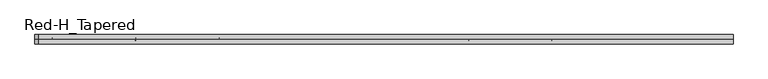
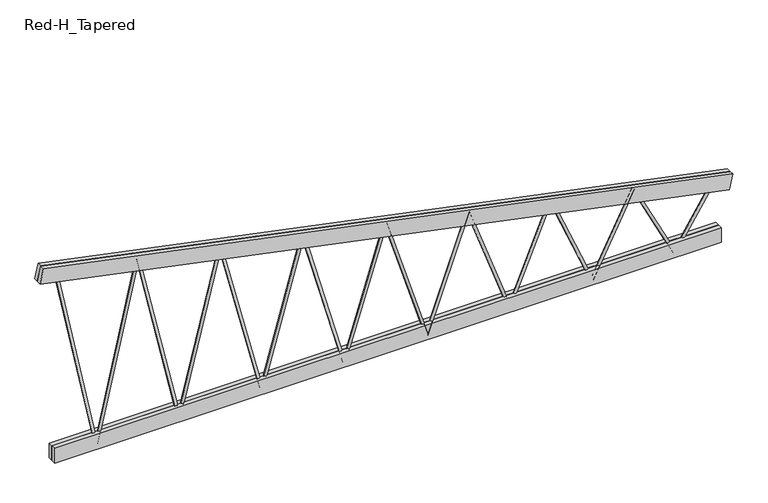
"""IFC4 building model written with IfcOpenShell, lengths in millimetres: beam geometry, Construction_Frames_RedBuilt_Openweb_Red-H_Tapered : Red-H_Tapered."""

from ifc_helpers import new_model, si_unit, point, frame, origin, origin_2d, place, context, project, spatial, polyline, circle_curve, trimmed, segment, composite_curve, outline, extrude, source, transform, mapped, element, save


def red_h_tapered_cb119500(model_context):
    return source(origin(), model_context, "Body", "SweptSolid", [
        extrude(outline(composite_curve([segment(trimmed(circle_curve(origin_2d(), 12.7), [point((0.0, 12.7))], [point((0.0, -12.7))], False, "CARTESIAN"), True, "CONTINUOUS"), segment(trimmed(circle_curve(origin_2d(), 12.7), [point((0.0, -12.7))], [point((0.0, 12.7))], False, "CARTESIAN"), True, "CONTINUOUS")], self_intersect=False)), frame((-368.7971472, 0.0, -367.0101562), z_axis=(-0.26750269153884754, 0.0, 0.9635571130034131), x_axis=(0.0, -1.0, 0.0)), (0.0, 0.0, 1.0), 1378.6670521),
        extrude(outline(composite_curve([segment(trimmed(circle_curve(origin_2d(), 12.7), [point((0.0, -12.7))], [point((0.0, 12.7))], False, "CARTESIAN"), True, "CONTINUOUS"), segment(trimmed(circle_curve(origin_2d(), 12.7), [point((0.0, 12.7))], [point((0.0, -12.7))], False, "CARTESIAN"), True, "CONTINUOUS")], self_intersect=False)), frame((-1106.3914415, 0.0, -367.0101562), z_axis=(0.2675026915388467, 0.0, 0.9635571130034134), x_axis=(0.0, -1.0, 0.0)), (0.0, 0.0, 1.0), 1378.6670521),
        extrude(outline(composite_curve([segment(trimmed(circle_curve(origin_2d(), 12.7), [point((0.0, 12.6999999))], [point((0.0, -12.7))], False, "CARTESIAN"), True, "CONTINUOUS"), segment(trimmed(circle_curve(origin_2d(), 12.7), [point((0.0, -12.7))], [point((0.0, 12.6999999))], False, "CARTESIAN"), True, "CONTINUOUS")], self_intersect=False)), frame((-1106.3914415, 0.0, -367.0101562), z_axis=(-0.2422140667731756, 0.0, 0.9702228330941298), x_axis=(0.0, -1.0, 0.0)), (0.0, 0.0, 1.0), 1522.6082948),
        extrude(outline(composite_curve([segment(trimmed(circle_curve(origin_2d(), 12.7), [point((0.0, -12.7))], [point((0.0, 12.7))], False, "CARTESIAN"), True, "CONTINUOUS"), segment(trimmed(circle_curve(origin_2d(), 12.7), [point((0.0, 12.7))], [point((0.0, -12.7))], False, "CARTESIAN"), True, "CONTINUOUS")], self_intersect=False)), frame((-1843.9857359, 0.0, -367.0101562), z_axis=(0.2422140667731837, 0.0, 0.9702228330941278), x_axis=(0.0, -1.0, 0.0)), (0.0, 0.0, 1.0), 1522.6082948),
        extrude(outline(composite_curve([segment(trimmed(circle_curve(origin_2d(), 12.7), [point((0.0, 12.7))], [point((0.0, -12.7))], False, "CARTESIAN"), True, "CONTINUOUS"), segment(trimmed(circle_curve(origin_2d(), 12.7), [point((0.0, -12.7))], [point((0.0, 12.7))], False, "CARTESIAN"), True, "CONTINUOUS")], self_intersect=False)), frame((-1843.9857359, 0.0, -367.0101562), z_axis=(-0.22117953511549954, 0.0, 0.9752331071318752), x_axis=(0.0, -1.0, 0.0)), (0.0, 0.0, 1.0), 1667.4108072),
        extrude(outline(composite_curve([segment(trimmed(circle_curve(origin_2d(), 12.7), [point((0.0, -12.6999999))], [point((0.0, 12.7))], False, "CARTESIAN"), True, "CONTINUOUS"), segment(trimmed(circle_curve(origin_2d(), 12.7), [point((0.0, 12.7))], [point((0.0, -12.6999999))], False, "CARTESIAN"), True, "CONTINUOUS")], self_intersect=False)), frame((-2581.5800303, 0.0, -367.0101562), z_axis=(0.22117953511549293, 0.0, 0.9752331071318767), x_axis=(0.0, -1.0, 0.0)), (0.0, 0.0, 1.0), 1667.4108072),
        extrude(outline(composite_curve([segment(trimmed(circle_curve(origin_2d(), 12.7), [point((0.0, 12.7))], [point((0.0, -12.7))], False, "CARTESIAN"), True, "CONTINUOUS"), segment(trimmed(circle_curve(origin_2d(), 12.7), [point((0.0, -12.7))], [point((0.0, 12.7))], False, "CARTESIAN"), True, "CONTINUOUS")], self_intersect=False)), frame((-2581.5800303, 0.0, -367.0101562), z_axis=(-0.2034329595212491, 0.0, 0.9790888779781056), x_axis=(0.0, -1.0, 0.0)), (0.0, 0.0, 1.0), 1812.8682198),
        extrude(outline(composite_curve([segment(trimmed(circle_curve(origin_2d(), 12.7), [point((0.0, 12.7))], [point((0.0, -12.7))], False, "CARTESIAN"), True, "CONTINUOUS"), segment(trimmed(circle_curve(origin_2d(), 12.7), [point((0.0, -12.7))], [point((0.0, 12.7))], False, "CARTESIAN"), True, "CONTINUOUS")], self_intersect=False)), frame((2581.5800303, 0.0, -367.0101562), z_axis=(0.5338157604547286, 0.0, 0.8456008123755203), x_axis=(0.0, -1.0, 0.0)), (0.0, 0.0, 1.0), 690.8697242),
        extrude(outline(composite_curve([segment(trimmed(circle_curve(origin_2d(), 12.7), [point((0.0, -12.7000001))], [point((0.0, 12.6999999))], False, "CARTESIAN"), True, "CONTINUOUS"), segment(trimmed(circle_curve(origin_2d(), 12.7), [point((0.0, 12.6999999))], [point((0.0, -12.7000001))], False, "CARTESIAN"), True, "CONTINUOUS")], self_intersect=False)), frame((2581.5800303, 0.0, -367.0101562), z_axis=(-0.4494298504402509, 0.0, 0.8933156270508502), x_axis=(0.0, -1.0, 0.0)), (0.0, 0.0, 1.0), 820.5889013),
        extrude(outline(composite_curve([segment(trimmed(circle_curve(origin_2d(), 12.7), [point((0.0, 12.7000001))], [point((0.0, -12.7))], False, "CARTESIAN"), True, "CONTINUOUS"), segment(trimmed(circle_curve(origin_2d(), 12.7), [point((0.0, -12.7))], [point((0.0, 12.7000001))], False, "CARTESIAN"), True, "CONTINUOUS")], self_intersect=False)), frame((1843.9857359, 0.0, -367.0101562), z_axis=(0.44942985044025024, 0.0, 0.8933156270508507), x_axis=(0.0, -1.0, 0.0)), (0.0, 0.0, 1.0), 820.5889013),
        extrude(outline(composite_curve([segment(trimmed(circle_curve(origin_2d(), 12.7), [point((0.0, -12.7))], [point((0.0, 12.7))], False, "CARTESIAN"), True, "CONTINUOUS"), segment(trimmed(circle_curve(origin_2d(), 12.7), [point((0.0, 12.7))], [point((0.0, -12.7))], False, "CARTESIAN"), True, "CONTINUOUS")], self_intersect=False)), frame((1843.9857359, 0.0, -367.0101562), z_axis=(-0.38581225339019065, 0.0, 0.9225773166157856), x_axis=(0.0, -1.0, 0.0)), (0.0, 0.0, 1.0), 955.8979632),
        extrude(outline(composite_curve([segment(trimmed(circle_curve(origin_2d(), 12.7), [point((0.0, 12.7000001))], [point((0.0, -12.7))], False, "CARTESIAN"), True, "CONTINUOUS"), segment(trimmed(circle_curve(origin_2d(), 12.7), [point((0.0, -12.7))], [point((0.0, 12.7000001))], False, "CARTESIAN"), True, "CONTINUOUS")], self_intersect=False)), frame((1106.3914415, 0.0, -367.0101562), z_axis=(0.38581225339018976, 0.0, 0.9225773166157859), x_axis=(0.0, -1.0, 0.0)), (0.0, 0.0, 1.0), 955.8979632),
        extrude(outline(composite_curve([segment(trimmed(circle_curve(origin_2d(), 12.7), [point((0.0, -12.7))], [point((0.0, 12.7))], False, "CARTESIAN"), True, "CONTINUOUS"), segment(trimmed(circle_curve(origin_2d(), 12.7), [point((0.0, 12.7))], [point((0.0, -12.7))], False, "CARTESIAN"), True, "CONTINUOUS")], self_intersect=False)), frame((1106.3914415, 0.0, -367.0101562), z_axis=(-0.3368853074093003, 0.0, 0.9415456917493391), x_axis=(0.0, -1.0, 0.0)), (0.0, 0.0, 1.0), 1094.7261251),
        extrude(outline(composite_curve([segment(trimmed(circle_curve(origin_2d(), 12.7), [point((0.0, 12.7))], [point((0.0, -12.7))], False, "CARTESIAN"), True, "CONTINUOUS"), segment(trimmed(circle_curve(origin_2d(), 12.7), [point((0.0, -12.7))], [point((0.0, 12.7))], False, "CARTESIAN"), True, "CONTINUOUS")], self_intersect=False)), frame((368.7971472, 0.0, -367.0101562), z_axis=(0.33688530740930067, 0.0, 0.9415456917493389), x_axis=(0.0, -1.0, 0.0)), (0.0, 0.0, 1.0), 1094.7261251),
        extrude(outline(composite_curve([segment(trimmed(circle_curve(origin_2d(), 12.7), [point((0.0, -12.7))], [point((0.0, 12.7))], False, "CARTESIAN"), True, "CONTINUOUS"), segment(trimmed(circle_curve(origin_2d(), 12.7), [point((0.0, 12.7))], [point((0.0, -12.7))], False, "CARTESIAN"), True, "CONTINUOUS")], self_intersect=False)), frame((368.7971472, 0.0, -367.0101562), z_axis=(-0.29840659773502576, 0.0, 0.9544388416384816), x_axis=(0.0, -1.0, 0.0)), (0.0, 0.0, 1.0), 1235.8880466),
        extrude(outline(composite_curve([segment(trimmed(circle_curve(origin_2d(), 12.7), [point((0.0, -12.7))], [point((0.0, 12.7))], False, "CARTESIAN"), True, "CONTINUOUS"), segment(trimmed(circle_curve(origin_2d(), 12.7), [point((0.0, 12.7))], [point((0.0, -12.7))], False, "CARTESIAN"), True, "CONTINUOUS")], self_intersect=False)), frame((-368.7971472, 0.0, -367.0101562), z_axis=(0.29840659773500394, 0.0, 0.9544388416384885), x_axis=(0.0, -1.0, 0.0)), (0.0, 0.0, 1.0), 1235.8880466),
        extrude(outline(polyline([(-2975.7771774, -41.275), (-2975.7771774, -3.175), (2975.7771774, -3.175), (2975.7771774, -41.275), (-2975.7771774, -41.275)])), frame((0.0, 0.0, -386.0601562), z_axis=(0.0, 0.0, 1.0), x_axis=(1.0, 0.0, 0.0)), (0.0, 0.0, 1.0), 139.7),
        extrude(outline(polyline([(-2975.7771774, 3.175), (-2975.7771774, 41.275), (2975.7771774, 41.275), (2975.7771774, 3.175), (-2975.7771774, 3.175)])), frame((0.0, 0.0, -386.0601562), z_axis=(0.0, 0.0, 1.0), x_axis=(1.0, 0.0, 0.0)), (0.0, 0.0, 1.0), 139.7),
        extrude(outline(polyline([(0.0, -38.1), (0.0, 0.0), (6282.8180718, 0.0), (6282.8180718, -38.1), (0.0, -38.1)])), frame((-3105.4394465, -3.175, 1348.7498719), z_axis=(0.20087522598673502, 0.0, 0.9796168350864425), x_axis=(0.9796168350864425, 0.0, -0.20087522598673502)), (0.0, 0.0, 1.0), 139.7),
        extrude(outline(polyline([(0.0, -38.1), (0.0, 0.0), (6282.8180718, 0.0), (6282.8180718, -38.1), (0.0, -38.1)])), frame((-3105.4394465, 41.275, 1348.7498719), z_axis=(0.20087522598673502, 0.0, 0.9796168350864425), x_axis=(0.9796168350864425, 0.0, -0.20087522598673502)), (0.0, 0.0, 1.0), 139.7),
    ])


if __name__ == "__main__":
    model = new_model("IFC4")
    model_context = context("Model", 3, world=origin())
    ifc_project = project(units=[si_unit("LENGTHUNIT", "METRE", prefix="MILLI")], contexts=[model_context])
    site = spatial("IfcSite", under=ifc_project)
    building = spatial("IfcBuilding", under=site)
    placement = place(None, origin())
    red_h_tapered_shape = red_h_tapered_cb119500(model_context)
    element("IfcBeam", 1, ObjectType="Construction_Frames_RedBuilt_Openweb_Red-H_Tapered : Red-H_Tapered", at=placement, inside=building, context=model_context, shape_type="MappedRepresentation", body=[
        mapped(red_h_tapered_shape, transform((0.0, 0.0, 0.0), x_axis=(1.0, 0.0, 0.0), y_axis=(0.0, 1.0, 0.0), z_axis=(0.0, 0.0, 1.0))),
    ])
    save(model, "model.ifc")

# Revit data of these elements
# Type "Construction_Frames_RedBuilt_Openweb_Red-H_Tapered : Red-H_Tapered"
#   Youtube clip = ""
#   Weight Net (Kg) = "0"
#   Webs = "Up to 2\" diameter tubular steel"
#   Uniformat II Description = ""
#   Uniformat II Code = ""
#   Uniclass 2015 Name = "Softwood trusses"
#   Uniclass 2015 Code = "Pr_20_85_90_81"
#   Uniclass 2.0 Description = "Structural Framing Systems"
#   Uniclass 2.0 Code = "SS-15-10-75"
#   Uniclass 1.4 Description = "Trusses"
#   Uniclass 1.4 Code = "L3523"
#   UNSPSC Code = "30103606"
#   Technical description = "http://www.redbuilt.com/reference/literature-and-other-resources"
#   Region South America = "None"
#   Region Oceania = "None"
#   Region North America = "US"
#   Region Middle East = "None"
#   Region Europe = "None"
#   Region Asia = "None"
#   Region Antarctica = "None"
#   Region Africa = "None"
#   QR code = "http://bimobject.com/redbuilt/product/redbuilt-0003"
#   Product url = "http://www.redbuilt.com/products/default.aspx?id=2"
#   Product group = "Wood Trusses"
#   Product family = "Construction"
#   Product data url = "https://bimobject.com/redbuilt/product/redbuilt-0003"
#   Product certification = ""
#   Product SKU = "redbuilt-0003"
#   Product Page URL = "http://www.redbuilt.com/commercial-systems/red-m-red-h-open-web-trusses"
#   Product Guid = "2c5793f2-6ffb-4665-b825-cf90c048e711"
#   Product Documentation Link = "http://www.redbuilt.com/documents/OW_Guide_2017_07_LowRes_wLinks.pdf"
#   OmniClass Description = "Wood Trusses"
#   OmniClass Code = "23-13 35 19 13 17"
#   NBS Reference Description = ""
#   NBS Reference Code = ""
#   Material secondary = "Steel"
#   Material main = "Wood"
#   Masterformat 2014 Description = "Metal-Web Wood Joists"
#   Masterformat 2014 Code = "06 17 36"
#   Manufacturer name = "RedBuilt"
#   Manufacturer country = "United States"
#   Installation instructions = "http://www.redbuilt.com/documents/Installation_Sheets_Open-Web.pdf"
#   IFC Classification = ""
#   EAN code = ""
#   Design country = "United States"
#   Product Information = "http://redbuilt.com/products/default.aspx?id=2"
#   Model = "Red-H-Tapered"
#   Manufacturer URL = "http://redbuilt.com/"
#   Manufacturer = "RedBuilt™"
#   Description = "Open Web Truss"
#   Date of publishing = "8/17/2010"
#   Contact us = "http://redbuilt.com/contact/"
#   Chords = "Double 1½\" x 5½\" MSR lumber"
#   COBIe Type Category = ""
#   Brand url = "http://www.redbuilt.com"
#   BIMobject main category code = "construction"
#   BIMobject main category = "Construction"
#   BIMobject category code = "construction-frames-trusses"
#   BIMobject category = "Frames & Trusses"
#   Web Radius = 0' - 0 1/2"
#   Web Layout Offset Start [instance default] = 0' - 5"
#   Web Layout Offset End [instance default] = 0' - 5"
#   Web Diameter = 0' - 1"
#   TotalLength [instance default] = 20' - 0"
#   Span Minimum = 4' - 0"
#   Span Maximum = 70' - 0"
#   Span Limit [instance default] = 20' - 0"
#   Nominal width = 0' - 0"
#   Nominal height = 0' - 0"
#   Inner Depth Top [instance default] = 0' - 2.76372"
#   Depth Start [instance default] = 6' - 0"
#   Top Chord Length [instance default] = 20' - 1.19701"
#   TC Extension Start Aux [instance default] = 0' - 0"
#   TC Extension End Aux [instance default] = 0' - 0"
#   T-B Chord Length Difference L [instance default] = 0' - 4"
#   T-B Chord Length Difference [instance default] = 0' - 4"
#   Height 2 [instance default] = 6' - 0"
#   Depth Minimum at Wall = 2' - 0"
#   Depth Maximum at Wall = 6' - 0"
#   Depth Lower End [instance default] = 2' - 0"
#   Depth Higher End [instance default] = 6' - 0"
#   Depth End [instance default] = 2' - 0"
#   Depth 2 [instance default] = 2' - 0"
#   Chord Width = 0' - 3 1/4"
#   Chord Thickness = 0' - 1 1/2"
#   Chord Depth = 0' - 5 1/2"
#   Offset Start [instance default] = 0' - 0"
#   TC Extension Start [instance default] = 0' - 0"
#   End Panel = 0' - 5"
#   Offset End [instance default] = 0' - 0"
#   TC Extension End [instance default] = 0' - 0"
#   Length [instance default] = 20' - 0"
#   Angle [instance default] = 5.71059°
#   Span Limit Warning [instance default] = no
#   Edition number = 1
#   Top Bearing Start [instance default] = yes
#   Top Bearing End [instance default] = yes
#   Bottom Bearing Start [instance default] = no
#   Bottom Bearing End [instance default] = no
#   8 Panels [instance default] = yes
#   16 Panels [instance default] = no
#   12 Panels [instance default] = no
#   Web Material = RedBuilt-Steel, Galvanized
#   Clip Material = RedBuilt-Steel, Galvanized
#   Chords Material = RedBuilt-MSR
#   URL = ""
#   Assembly Code = ""
# Element 1 (IfcBeam, "Construction_Frames_RedBuilt_Openweb_Red-H_Tapered : Red-H_Tapered")
#   TotalLength = 20' - 2.31316"
#   Span Limit = 20' - 2.31316"
#   Inner Depth Top = 0' - 2.80722"
#   Top Chord Length = 20' - 7.35504"
#   Depth 2 = 4' - 1 11/16"
#   Angle = 11.5881°
#   Materials on its faces: "RedBuilt-Steel, Galvanized", "RedBuilt-MSR"
# Materials
#   "RedBuilt-Steel, Galvanized": class "Metal", colour RGB 164 172 176, transparency 0, Manufacturer = "RedBuilt. LLC", Comments = "Openweb Metal Web", URL = "http://www.redbuilt.com/", Description = "Galvanized steel", Cost = 0
#   "RedBuilt-MSR": class "Wood", colour RGB 213 182 136, transparency 0, Manufacturer = "RedBuilt, LLC", URL = "http://www.redbuilt.com/", Cost = 0
